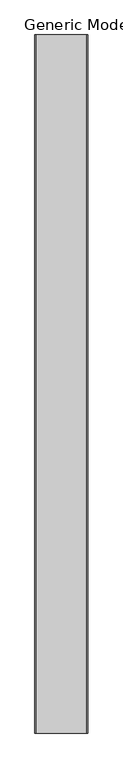
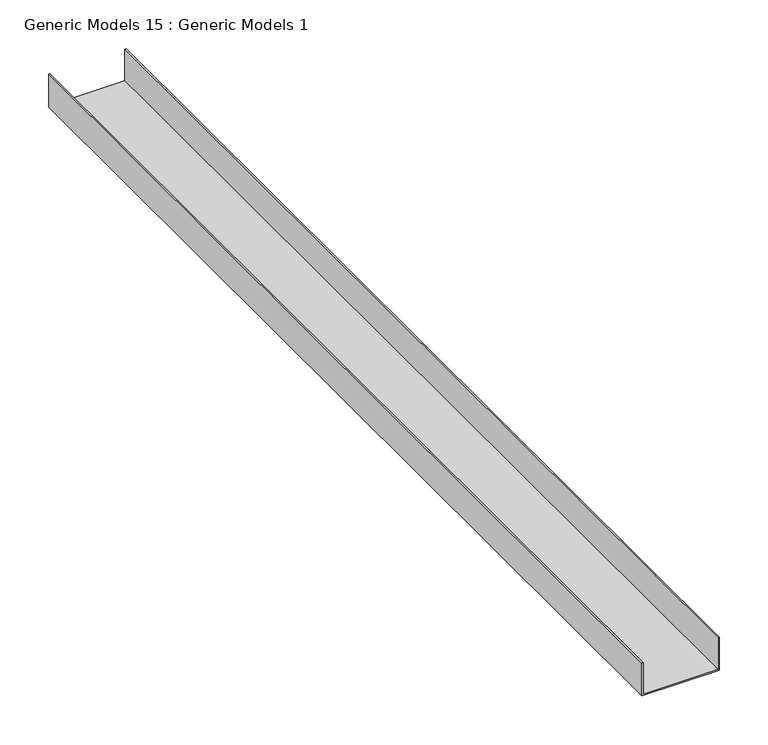
"""IFC4 building model written with IfcOpenShell, lengths in millimetres: proxy geometry, Generic Models 15 : Generic Models 1."""

import ifcopenshell
import ifcopenshell.guid

model = None  # the IFC model being written
_history = None  # IfcOwnerHistory: only IFC2X3 demands one
_inside = {}  # id of a spatial element -> (the spatial element, [elements in it])
_under = {}  # id of a project, library or spatial element -> (it, [spatial elements below it])
_declared = {}  # id of a project -> (the project, [libraries it declares])
_typed = {}  # id of a type object -> (the type object, [elements of that type])
_made_of = {}  # id of a material, layer set ... -> (it, [elements and type objects made of it])


def new_model(schema):
    """Start an empty IFC model of exactly this schema.

    Asked for "IFC4X3", IfcOpenShell would pick the latest addendum, in which some entities
    have other attributes; the version numbers below select the first issue.
    IFC2X3 requires an IfcOwnerHistory on every rooted entity: one is made here for all.
    """
    global model, _history
    if schema == "IFC4X3":
        model = ifcopenshell.file(schema_version=(4, 3, 0, 0))
    else:
        model = ifcopenshell.file(schema=schema)
    _inside.clear()
    _under.clear()
    _declared.clear()
    _typed.clear()
    _made_of.clear()
    _history = None
    if model.schema == "IFC2X3":
        org = make("IfcOrganization", Name="unknown")
        user = make(
            "IfcPersonAndOrganization",
            ThePerson=make("IfcPerson", FamilyName="unknown"),
            TheOrganization=org,
        )
        app = make(
            "IfcApplication",
            ApplicationDeveloper=org,
            Version="unknown",
            ApplicationFullName="unknown",
            ApplicationIdentifier="unknown",
        )
        _history = make(
            "IfcOwnerHistory",
            OwningUser=user,
            OwningApplication=app,
            ChangeAction="ADDED",
            CreationDate=0,
        )
    return model


def make(cls, **values):
    """One entity of the class cls with the attributes given. An attribute that is None is left unset."""
    return model.create_entity(
        cls, **{name: value for name, value in values.items() if value is not None}
    )


def rooted(cls, **values):
    """An entity with a GlobalId (a new one), such as an element, a storey or a relation."""
    return make(cls, GlobalId=ifcopenshell.guid.new(), OwnerHistory=_history, **values)


def si_unit(unit_type, name, prefix=None):
    """IfcSIUnit, for example si_unit("LENGTHUNIT", "METRE", prefix="MILLI")."""
    return make("IfcSIUnit", UnitType=unit_type, Prefix=prefix, Name=name)


def assignment(units):
    """IfcUnitAssignment: the units of a project."""
    return None if units is None else make("IfcUnitAssignment", Units=units)


def point(xyz):
    """IfcCartesianPoint."""
    return None if xyz is None else make("IfcCartesianPoint", Coordinates=xyz)


def direction(xyz):
    """IfcDirection."""
    return None if xyz is None else make("IfcDirection", DirectionRatios=xyz)


def frame(location, z_axis=None, x_axis=None):
    """IfcAxis2Placement3D, a coordinate frame: its origin and axes. An axis left out is left unset."""
    return make(
        "IfcAxis2Placement3D",
        Location=point(location),
        Axis=direction(z_axis),
        RefDirection=direction(x_axis),
    )


def origin():
    """The frame at (0, 0, 0) with its axes left unset."""
    return frame((0.0, 0.0, 0.0))


def place(relative_to, where):
    """IfcLocalPlacement: puts the frame where relative to a parent placement (None: the world)."""
    return make(
        "IfcLocalPlacement", PlacementRelTo=relative_to, RelativePlacement=where
    )


def context(
    kind, dimensions, precision=None, world=None, true_north=None, identifier=None
):
    """IfcGeometricRepresentationContext, for example the 3D "Model" context."""
    return make(
        "IfcGeometricRepresentationContext",
        ContextIdentifier=identifier,
        ContextType=kind,
        CoordinateSpaceDimension=dimensions,
        Precision=precision,
        WorldCoordinateSystem=world,
        TrueNorth=true_north,
    )


def project(units=None, contexts=None):
    """IfcProject with its units and contexts."""
    return rooted(
        "IfcProject",
        Name="project",
        RepresentationContexts=contexts,
        UnitsInContext=assignment(units),
    )


def spatial(cls, under=None, at=None, **own):
    """A site, building, storey or space (cls), placed at a placement, below another one or the project."""
    s = rooted(cls, ObjectPlacement=at, **own)
    if under is not None:
        _under.setdefault(under.id(), (under, []))[1].append(s)
    return s


def polyline(points):
    """IfcPolyline through the points."""
    return make("IfcPolyline", Points=[point(p) for p in points])


def outline(outer, holes=None, kind="AREA"):
    """IfcArbitraryClosedProfileDef: a profile drawn as a closed curve; with holes, ...WithVoids."""
    if holes is None:
        return make("IfcArbitraryClosedProfileDef", ProfileType=kind, OuterCurve=outer)
    return make(
        "IfcArbitraryProfileDefWithVoids",
        ProfileType=kind,
        OuterCurve=outer,
        InnerCurves=holes,
    )


def extrude(swept, where, along, depth):
    """IfcExtrudedAreaSolid: the profile swept, set in the frame where, extruded along a direction by depth."""
    return make(
        "IfcExtrudedAreaSolid",
        SweptArea=swept,
        Position=where,
        ExtrudedDirection=direction(along),
        Depth=depth,
    )


def shape(context_of_items, identifier, shape_type, items):
    """IfcShapeRepresentation: the items that make up one representation, for example the "Body"."""
    return make(
        "IfcShapeRepresentation",
        ContextOfItems=context_of_items,
        RepresentationIdentifier=identifier,
        RepresentationType=shape_type,
        Items=items,
    )


def source(mapping_origin, context_of_items, identifier, shape_type, items):
    """IfcRepresentationMap: a shape defined once, which mapped items show again and again."""
    return make(
        "IfcRepresentationMap",
        MappingOrigin=mapping_origin,
        MappedRepresentation=shape(context_of_items, identifier, shape_type, items),
    )


def transform(
    local_origin,
    x_axis=None,
    y_axis=None,
    z_axis=None,
    scale=None,
    scale2=None,
    scale3=None,
    uniform=True,
):
    """IfcCartesianTransformationOperator3D, or its non-uniform kind. x_axis, y_axis, z_axis: its Axis1, 2, 3."""
    if uniform:
        return make(
            "IfcCartesianTransformationOperator3D",
            Axis1=direction(x_axis),
            Axis2=direction(y_axis),
            LocalOrigin=point(local_origin),
            Scale=scale,
            Axis3=direction(z_axis),
        )
    return make(
        "IfcCartesianTransformationOperator3DnonUniform",
        Axis1=direction(x_axis),
        Axis2=direction(y_axis),
        LocalOrigin=point(local_origin),
        Scale=scale,
        Axis3=direction(z_axis),
        Scale2=scale2,
        Scale3=scale3,
    )


def mapped(mapping_source, mapping_target):
    """IfcMappedItem: shows the shape of a source again, moved by a transform."""
    return make(
        "IfcMappedItem", MappingSource=mapping_source, MappingTarget=mapping_target
    )


def made_of(thing, what):
    """Note that an element or type object is made of a material, layer set ...; save() writes the relation."""
    if what is not None:
        _made_of.setdefault(what.id(), (what, []))[1].append(thing)
    return thing


def element(
    cls,
    number,
    at=None,
    inside=None,
    cuts=None,
    type_object=None,
    material=None,
    context=None,
    identifier="Body",
    shape_type=None,
    held_by="IfcProductDefinitionShape",
    body=None,
    shapes=None,
    **own,
):
    """One element of the class cls, such as IfcWall. Its Tag is "e" and its number.

    at: its placement. inside: the storey or other place that contains it. cuts: it is an
    opening in that element (IfcRelVoidsElement). A single representation is given by context,
    identifier, shape_type and body (its items); several are given by shapes. held_by: the class
    of the entity that holds the representations. save() writes the other relations.
    """
    e = rooted(cls, Tag="e%d" % number, ObjectPlacement=at, **own)
    if body is not None:
        shapes = [shape(context, identifier, shape_type, body)]
    if shapes is not None:
        e.Representation = make(held_by, Representations=shapes)
    if inside is not None:
        _inside.setdefault(inside.id(), (inside, []))[1].append(e)
    if cuts is not None:
        rooted(
            "IfcRelVoidsElement", RelatingBuildingElement=cuts, RelatedOpeningElement=e
        )
    if type_object is not None:
        _typed.setdefault(type_object.id(), (type_object, []))[1].append(e)
    return made_of(e, material)


def aggregate(whole, parts):
    """IfcRelAggregates: a whole, such as a stair, and the parts it consists of."""
    return rooted("IfcRelAggregates", RelatingObject=whole, RelatedObjects=parts)


def save(model, path):
    """Write the relations noted so far, then the file.

    IfcRelAggregates (storeys below a building ...), IfcRelContainedInSpatialStructure (elements
    in a storey), IfcRelDefinesByType, IfcRelAssociatesMaterial and IfcRelDeclares: one each for
    every whole, place, type object, material and project.
    """
    for whole, parts in _under.values():
        aggregate(whole, parts)
    for where, things in _inside.values():
        rooted(
            "IfcRelContainedInSpatialStructure",
            RelatedElements=things,
            RelatingStructure=where,
        )
    for kind, things in _typed.values():
        rooted("IfcRelDefinesByType", RelatedObjects=things, RelatingType=kind)
    for what, things in _made_of.values():
        rooted("IfcRelAssociatesMaterial", RelatedObjects=things, RelatingMaterial=what)
    for by, libraries in _declared.values():
        rooted("IfcRelDeclares", RelatingContext=by, RelatedDefinitions=libraries)
    model.write(path)


def generic_models_15_generic_models_1_38d4618c(model_context):
    return source(origin(), model_context, "Body", "SweptSolid", [
        extrude(outline(polyline([(0.0, 49784.0), (41.275, 49784.0), (41.275, 49782.4125), (1.5875, 49782.4125), (1.5875, 49693.5125), (41.275, 49693.5125), (41.275, 49691.925), (0.0, 49691.925), (0.0, 49784.0)])), frame((0.0, 0.0, 0.0), z_axis=(0.0, 1.0, 0.0), x_axis=(0.0, 0.0, 1.0)), (0.0, 0.0, 1.0), 1219.2),
    ])


if __name__ == "__main__":
    model = new_model("IFC4")
    model_context = context("Model", 3, world=origin())
    ifc_project = project(units=[si_unit("LENGTHUNIT", "METRE", prefix="MILLI")], contexts=[model_context])
    site = spatial("IfcSite", under=ifc_project)
    building = spatial("IfcBuilding", under=site)
    placement = place(None, origin())
    generic_models_15_generic_models_1_shape = generic_models_15_generic_models_1_38d4618c(model_context)
    element("IfcBuildingElementProxy", 1, Name="Generic Models 15 : Generic Models 1", ObjectType="Generic Models 15 : Generic Models 1", at=placement, inside=building, context=model_context, shape_type="MappedRepresentation", body=[
        mapped(generic_models_15_generic_models_1_shape, transform((0.0, 0.0, 0.0), x_axis=(1.0, 0.0, 0.0), y_axis=(0.0, 1.0, 0.0), z_axis=(0.0, 0.0, 1.0))),
    ])
    save(model, "model.ifc")

# Revit data of these elements
# Element 1 (IfcBuildingElementProxy, "Generic Models 15 : Generic Models 1")
#   Materials on its faces: "METAL RUNNER CHANNEL; FASTEN @ 24\" O.C."
# Materials
#   "METAL RUNNER CHANNEL; FASTEN @ 24\" O.C.": class "Unassigned", colour RGB 210 209 208, transparency 0, Keynote = "M05121300.02", Cost = 0
